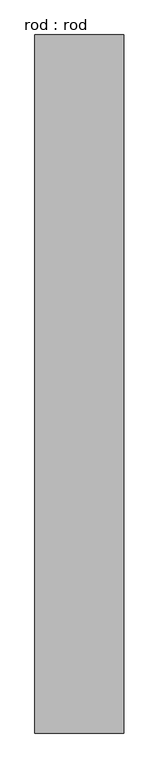
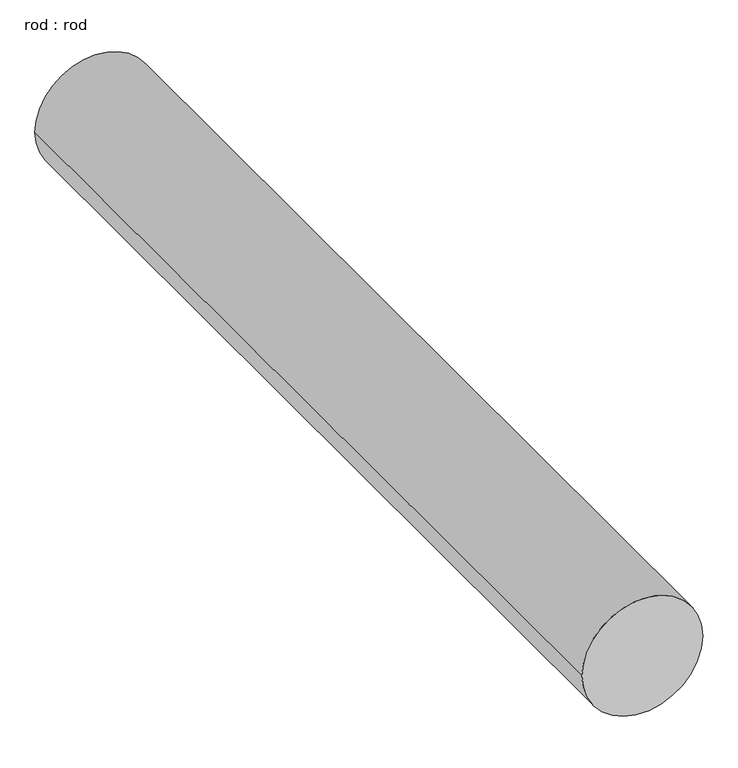
"""IFC4 building model written with IfcOpenShell, lengths in millimetres: proxy geometry, rod : rod."""

from ifc_helpers import new_model, si_unit, point, frame, frame_2d, origin, place, context, project, spatial, circle_curve, trimmed, segment, composite_curve, outline, extrude, source, transform, mapped, element, save


def rod_rod_12e0c67a(model_context):
    return source(origin(), model_context, "Body", "SweptSolid", [
        extrude(outline(composite_curve([segment(trimmed(circle_curve(frame_2d((0.0108462, 0.0)), 200.0), [point((0.0108462, 200.0))], [point((0.0108462, -200.0))], False, "CARTESIAN"), True, "CONTINUOUS"), segment(trimmed(circle_curve(frame_2d((0.0108462, 0.0)), 200.0), [point((0.0108462, -200.0))], [point((0.0108462, 200.0))], False, "CARTESIAN"), True, "CONTINUOUS")], self_intersect=False)), frame((0.0, 2523.0857582, 0.0), z_axis=(0.0, 1.0, 0.0), x_axis=(0.0, 0.0, 1.0)), (0.0, 0.0, 1.0), 3139.2857143),
    ])


if __name__ == "__main__":
    model = new_model("IFC4")
    model_context = context("Model", 3, world=origin())
    ifc_project = project(units=[si_unit("LENGTHUNIT", "METRE", prefix="MILLI")], contexts=[model_context])
    site = spatial("IfcSite", under=ifc_project)
    building = spatial("IfcBuilding", under=site)
    placement = place(None, origin())
    rod_rod_shape = rod_rod_12e0c67a(model_context)
    element("IfcBuildingElementProxy", 1, Name="rod : rod", ObjectType="rod : rod", at=placement, inside=building, context=model_context, shape_type="MappedRepresentation", body=[
        mapped(rod_rod_shape, transform((0.0, 0.0, 0.0), x_axis=(1.0, 0.0, 0.0), y_axis=(0.0, 1.0, 0.0), z_axis=(0.0, 0.0, 1.0))),
    ])
    save(model, "model.ifc")

# Revit data of these elements
# Type "rod : rod"
#   Default Elevation = 0
